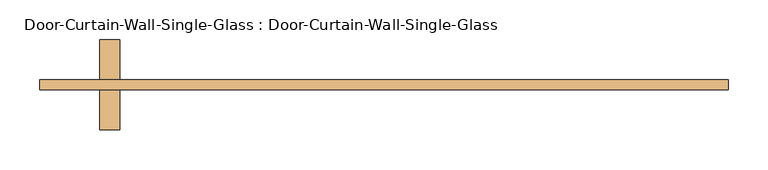
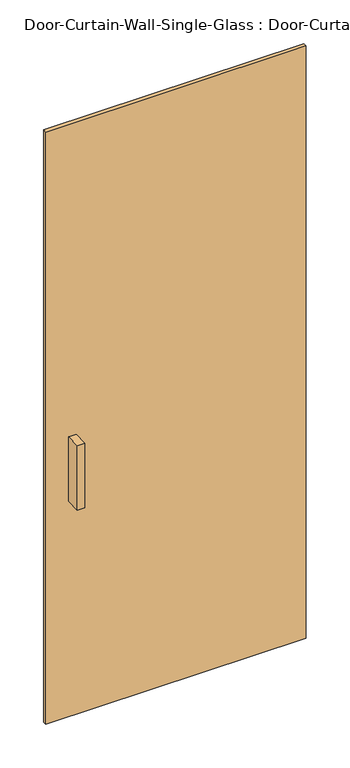
"""IFC4 building model written with IfcOpenShell, lengths in millimetres: door geometry, Door-Curtain-Wall-Single-Glass : Door-Curtain-Wall-Single-Glass."""

import ifcopenshell
import ifcopenshell.guid

model = None  # the IFC model being written
_history = None  # IfcOwnerHistory: only IFC2X3 demands one
_inside = {}  # id of a spatial element -> (the spatial element, [elements in it])
_under = {}  # id of a project, library or spatial element -> (it, [spatial elements below it])
_declared = {}  # id of a project -> (the project, [libraries it declares])
_typed = {}  # id of a type object -> (the type object, [elements of that type])
_made_of = {}  # id of a material, layer set ... -> (it, [elements and type objects made of it])


def new_model(schema):
    """Start an empty IFC model of exactly this schema.

    Asked for "IFC4X3", IfcOpenShell would pick the latest addendum, in which some entities
    have other attributes; the version numbers below select the first issue.
    IFC2X3 requires an IfcOwnerHistory on every rooted entity: one is made here for all.
    """
    global model, _history
    if schema == "IFC4X3":
        model = ifcopenshell.file(schema_version=(4, 3, 0, 0))
    else:
        model = ifcopenshell.file(schema=schema)
    _inside.clear()
    _under.clear()
    _declared.clear()
    _typed.clear()
    _made_of.clear()
    _history = None
    if model.schema == "IFC2X3":
        org = make("IfcOrganization", Name="unknown")
        user = make(
            "IfcPersonAndOrganization",
            ThePerson=make("IfcPerson", FamilyName="unknown"),
            TheOrganization=org,
        )
        app = make(
            "IfcApplication",
            ApplicationDeveloper=org,
            Version="unknown",
            ApplicationFullName="unknown",
            ApplicationIdentifier="unknown",
        )
        _history = make(
            "IfcOwnerHistory",
            OwningUser=user,
            OwningApplication=app,
            ChangeAction="ADDED",
            CreationDate=0,
        )
    return model


def make(cls, **values):
    """One entity of the class cls with the attributes given. An attribute that is None is left unset."""
    return model.create_entity(
        cls, **{name: value for name, value in values.items() if value is not None}
    )


def rooted(cls, **values):
    """An entity with a GlobalId (a new one), such as an element, a storey or a relation."""
    return make(cls, GlobalId=ifcopenshell.guid.new(), OwnerHistory=_history, **values)


def si_unit(unit_type, name, prefix=None):
    """IfcSIUnit, for example si_unit("LENGTHUNIT", "METRE", prefix="MILLI")."""
    return make("IfcSIUnit", UnitType=unit_type, Prefix=prefix, Name=name)


def assignment(units):
    """IfcUnitAssignment: the units of a project."""
    return None if units is None else make("IfcUnitAssignment", Units=units)


def point(xyz):
    """IfcCartesianPoint."""
    return None if xyz is None else make("IfcCartesianPoint", Coordinates=xyz)


def direction(xyz):
    """IfcDirection."""
    return None if xyz is None else make("IfcDirection", DirectionRatios=xyz)


def frame(location, z_axis=None, x_axis=None):
    """IfcAxis2Placement3D, a coordinate frame: its origin and axes. An axis left out is left unset."""
    return make(
        "IfcAxis2Placement3D",
        Location=point(location),
        Axis=direction(z_axis),
        RefDirection=direction(x_axis),
    )


def origin():
    """The frame at (0, 0, 0) with its axes left unset."""
    return frame((0.0, 0.0, 0.0))


def origin_with_axes():
    """The frame at (0, 0, 0) with the z axis (0, 0, 1) and the x axis (1, 0, 0) written out."""
    return frame((0.0, 0.0, 0.0), z_axis=(0.0, 0.0, 1.0), x_axis=(1.0, 0.0, 0.0))


def place(relative_to, where):
    """IfcLocalPlacement: puts the frame where relative to a parent placement (None: the world)."""
    return make(
        "IfcLocalPlacement", PlacementRelTo=relative_to, RelativePlacement=where
    )


def context(
    kind, dimensions, precision=None, world=None, true_north=None, identifier=None
):
    """IfcGeometricRepresentationContext, for example the 3D "Model" context."""
    return make(
        "IfcGeometricRepresentationContext",
        ContextIdentifier=identifier,
        ContextType=kind,
        CoordinateSpaceDimension=dimensions,
        Precision=precision,
        WorldCoordinateSystem=world,
        TrueNorth=true_north,
    )


def project(units=None, contexts=None):
    """IfcProject with its units and contexts."""
    return rooted(
        "IfcProject",
        Name="project",
        RepresentationContexts=contexts,
        UnitsInContext=assignment(units),
    )


def spatial(cls, under=None, at=None, **own):
    """A site, building, storey or space (cls), placed at a placement, below another one or the project."""
    s = rooted(cls, ObjectPlacement=at, **own)
    if under is not None:
        _under.setdefault(under.id(), (under, []))[1].append(s)
    return s


def polyline(points):
    """IfcPolyline through the points."""
    return make("IfcPolyline", Points=[point(p) for p in points])


def outline(outer, holes=None, kind="AREA"):
    """IfcArbitraryClosedProfileDef: a profile drawn as a closed curve; with holes, ...WithVoids."""
    if holes is None:
        return make("IfcArbitraryClosedProfileDef", ProfileType=kind, OuterCurve=outer)
    return make(
        "IfcArbitraryProfileDefWithVoids",
        ProfileType=kind,
        OuterCurve=outer,
        InnerCurves=holes,
    )


def extrude(swept, where, along, depth):
    """IfcExtrudedAreaSolid: the profile swept, set in the frame where, extruded along a direction by depth."""
    return make(
        "IfcExtrudedAreaSolid",
        SweptArea=swept,
        Position=where,
        ExtrudedDirection=direction(along),
        Depth=depth,
    )


def shape(context_of_items, identifier, shape_type, items):
    """IfcShapeRepresentation: the items that make up one representation, for example the "Body"."""
    return make(
        "IfcShapeRepresentation",
        ContextOfItems=context_of_items,
        RepresentationIdentifier=identifier,
        RepresentationType=shape_type,
        Items=items,
    )


def source(mapping_origin, context_of_items, identifier, shape_type, items):
    """IfcRepresentationMap: a shape defined once, which mapped items show again and again."""
    return make(
        "IfcRepresentationMap",
        MappingOrigin=mapping_origin,
        MappedRepresentation=shape(context_of_items, identifier, shape_type, items),
    )


def transform(
    local_origin,
    x_axis=None,
    y_axis=None,
    z_axis=None,
    scale=None,
    scale2=None,
    scale3=None,
    uniform=True,
):
    """IfcCartesianTransformationOperator3D, or its non-uniform kind. x_axis, y_axis, z_axis: its Axis1, 2, 3."""
    if uniform:
        return make(
            "IfcCartesianTransformationOperator3D",
            Axis1=direction(x_axis),
            Axis2=direction(y_axis),
            LocalOrigin=point(local_origin),
            Scale=scale,
            Axis3=direction(z_axis),
        )
    return make(
        "IfcCartesianTransformationOperator3DnonUniform",
        Axis1=direction(x_axis),
        Axis2=direction(y_axis),
        LocalOrigin=point(local_origin),
        Scale=scale,
        Axis3=direction(z_axis),
        Scale2=scale2,
        Scale3=scale3,
    )


def mapped(mapping_source, mapping_target):
    """IfcMappedItem: shows the shape of a source again, moved by a transform."""
    return make(
        "IfcMappedItem", MappingSource=mapping_source, MappingTarget=mapping_target
    )


def made_of(thing, what):
    """Note that an element or type object is made of a material, layer set ...; save() writes the relation."""
    if what is not None:
        _made_of.setdefault(what.id(), (what, []))[1].append(thing)
    return thing


def element(
    cls,
    number,
    at=None,
    inside=None,
    cuts=None,
    type_object=None,
    material=None,
    context=None,
    identifier="Body",
    shape_type=None,
    held_by="IfcProductDefinitionShape",
    body=None,
    shapes=None,
    **own,
):
    """One element of the class cls, such as IfcWall. Its Tag is "e" and its number.

    at: its placement. inside: the storey or other place that contains it. cuts: it is an
    opening in that element (IfcRelVoidsElement). A single representation is given by context,
    identifier, shape_type and body (its items); several are given by shapes. held_by: the class
    of the entity that holds the representations. save() writes the other relations.
    """
    e = rooted(cls, Tag="e%d" % number, ObjectPlacement=at, **own)
    if body is not None:
        shapes = [shape(context, identifier, shape_type, body)]
    if shapes is not None:
        e.Representation = make(held_by, Representations=shapes)
    if inside is not None:
        _inside.setdefault(inside.id(), (inside, []))[1].append(e)
    if cuts is not None:
        rooted(
            "IfcRelVoidsElement", RelatingBuildingElement=cuts, RelatedOpeningElement=e
        )
    if type_object is not None:
        _typed.setdefault(type_object.id(), (type_object, []))[1].append(e)
    return made_of(e, material)


def aggregate(whole, parts):
    """IfcRelAggregates: a whole, such as a stair, and the parts it consists of."""
    return rooted("IfcRelAggregates", RelatingObject=whole, RelatedObjects=parts)


def save(model, path):
    """Write the relations noted so far, then the file.

    IfcRelAggregates (storeys below a building ...), IfcRelContainedInSpatialStructure (elements
    in a storey), IfcRelDefinesByType, IfcRelAssociatesMaterial and IfcRelDeclares: one each for
    every whole, place, type object, material and project.
    """
    for whole, parts in _under.values():
        aggregate(whole, parts)
    for where, things in _inside.values():
        rooted(
            "IfcRelContainedInSpatialStructure",
            RelatedElements=things,
            RelatingStructure=where,
        )
    for kind, things in _typed.values():
        rooted("IfcRelDefinesByType", RelatedObjects=things, RelatingType=kind)
    for what, things in _made_of.values():
        rooted("IfcRelAssociatesMaterial", RelatedObjects=things, RelatingMaterial=what)
    for by, libraries in _declared.values():
        rooted("IfcRelDeclares", RelatingContext=by, RelatedDefinitions=libraries)
    model.write(path)


def door_curtain_wall_single_glass_door_curtain_wall_single_9586b40b(model_context):
    return source(origin(), model_context, "Body", "SweptSolid", [
        extrude(outline(polyline([(435.9649128, 0.0), (-435.9649128, 0.0), (-435.9649128, 12.7), (435.9649128, 12.7), (435.9649128, 0.0)])), origin_with_axes(), (0.0, 0.0, 1.0), 2095.5),
        extrude(outline(polyline([(-334.3649128, 63.5), (-334.3649128, 12.7), (-359.7649128, 12.7), (-359.7649128, 63.5), (-334.3649128, 63.5)])), frame((0.0, 0.0, 762.0), z_axis=(0.0, 0.0, 1.0), x_axis=(1.0, 0.0, 0.0)), (0.0, 0.0, 1.0), 228.6),
        extrude(outline(polyline([(-359.7649128, -50.8), (-359.7649128, 0.0), (-334.3649128, 0.0), (-334.3649128, -50.8), (-359.7649128, -50.8)])), frame((0.0, 0.0, 762.0), z_axis=(0.0, 0.0, 1.0), x_axis=(1.0, 0.0, 0.0)), (0.0, 0.0, 1.0), 228.6),
    ])


if __name__ == "__main__":
    model = new_model("IFC4")
    model_context = context("Model", 3, world=origin())
    ifc_project = project(units=[si_unit("LENGTHUNIT", "METRE", prefix="MILLI")], contexts=[model_context])
    site = spatial("IfcSite", under=ifc_project)
    building = spatial("IfcBuilding", under=site)
    placement = place(None, origin())
    door_curtain_wall_single_glass_door_curtain_wall_single_shape = door_curtain_wall_single_glass_door_curtain_wall_single_9586b40b(model_context)
    element("IfcDoor", 1, ObjectType="Door-Curtain-Wall-Single-Glass : Door-Curtain-Wall-Single-Glass", at=placement, inside=building, context=model_context, shape_type="MappedRepresentation", body=[
        mapped(door_curtain_wall_single_glass_door_curtain_wall_single_shape, transform((0.0, 0.0, 0.0), x_axis=(1.0, 0.0, 0.0), y_axis=(0.0, 1.0, 0.0), z_axis=(0.0, 0.0, 1.0))),
    ])
    save(model, "model.ifc")

# Revit data of these elements
# Type "Door-Curtain-Wall-Single-Glass : Door-Curtain-Wall-Single-Glass"
#   Type Mark = "9"
#   Assembly Code = "B2030100"
#   Analytic Construction = "<None>"
#   Width [instance default] = 3' - 0"
#   Thermal Resistance (R) = 10.0000 (h·ft²·°F)/BTU
#   Swing Angle [instance default] = 90.00°
#   Heat Transfer Coefficient (U) = 0.1000 BTU/(h·ft²·°F)
#   Offset = 0' - 0"
#   Define Thermal Properties by = 1
#   Function = 1
#   Door Handle Material = Aluminum
#   Glazing = Glass
#   Visual Light Transmittance = 0
#   Solar Heat Gain Coefficient = 0
#   Construction Type Id = ""
# Element 1 (IfcDoor, "Door-Curtain-Wall-Single-Glass : Door-Curtain-Wall-Single-Glass")
#   Width = 2' - 10.32795"
#   Materials on its faces: "Aluminum", "Glass"
# Materials
#   "Aluminum": class "Metal", colour RGB 247 247 247, transparency 0, Description = "Aluminum 6061", Cost = 0
#   "Glass": class "Glass", colour RGB 0 128 192, transparency 0.75, Description = "Soda Lime Glass", Cost = 0
